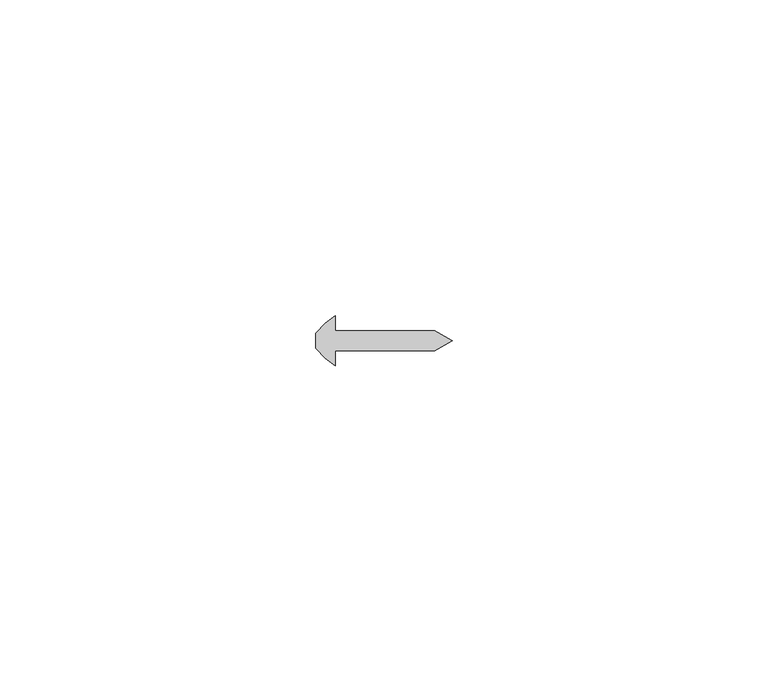
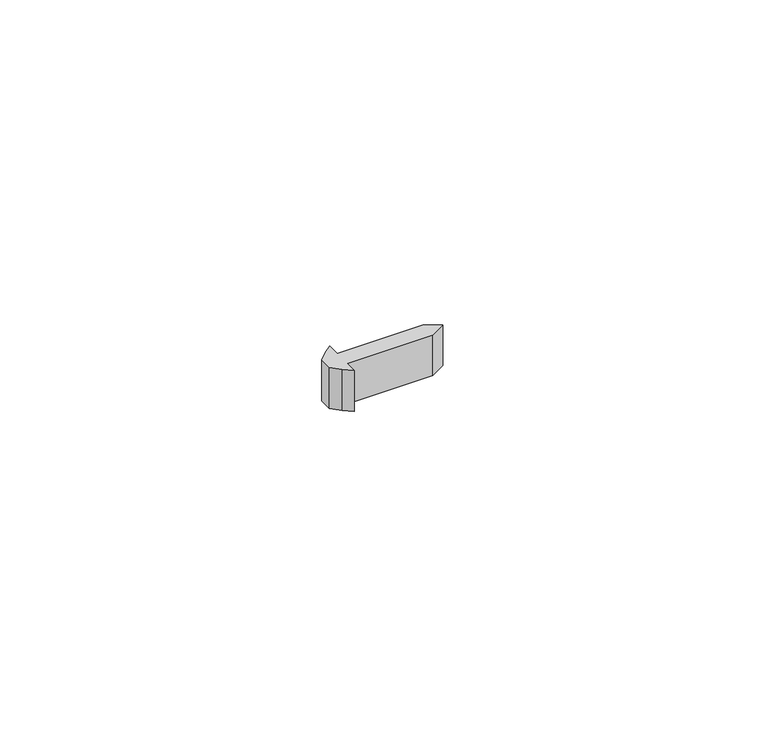
"""IFC4 building model written with IfcOpenShell, lengths in millimetres: proxy geometry, Generic Models 7:Generic Models 1:3:Generic Models 1:3 : Generic Models 7:Generic Models 1:305549:3:Generic Models 1:3:Generic Models 1:3 : Generic Models 7:Generic Models 1:305549:3 : Generic Models 7:Generic Models 1:3:Generic Models 1:3 : Generic Models 7:Generic Models 1:305549:301244:67 : Generic Models 7:Generic Models 1:3:Generic Models 1:3 : Generic Models 7:Generic Models 1:305549:3:Generic Models 1:3:Generic Models 1:3 : Generic Models 7:Generic Models 1:305549:3 : Generic Models 7:Generic Models 1:3:Generic Models 1:3 : Generic Models 7:Generic Models 1:305549:301244:308848."""

from ifc_helpers import new_model, si_unit, frame, origin, place, context, project, spatial, polyline, outline, extrude, source, transform, mapped, element, save


def generic_models_e5c60fd0(model_context):
    return source(origin(), model_context, "Body", "SweptSolid", [
        extrude(outline(polyline([(560281.5242239, -530659.7288841), (560281.5242239, -530662.1101341), (560279.9971659, -530660.8919386), (560278.4452757, -530659.3400484), (560278.4452757, -530656.9427199), (560279.9971659, -530655.3908297), (560281.5242239, -530654.1726341), (560281.5242239, -530656.5538841), (560297.3334794, -530656.5538841), (560300.0831101, -530658.1413841), (560297.3334794, -530659.7288841), (560281.5242239, -530659.7288841)])), frame((0.0, 0.0, 1237.45625), z_axis=(0.0, 0.0, 1.0), x_axis=(1.0, 0.0, 0.0)), (0.0, 0.0, 1.0), 7.9375),
    ])


if __name__ == "__main__":
    model = new_model("IFC4")
    model_context = context("Model", 3, world=origin())
    ifc_project = project(units=[si_unit("LENGTHUNIT", "METRE", prefix="MILLI")], contexts=[model_context])
    site = spatial("IfcSite", under=ifc_project)
    building = spatial("IfcBuilding", under=site)
    placement = place(None, origin())
    generic_models_shape = generic_models_e5c60fd0(model_context)
    element("IfcBuildingElementProxy", 1, Name="Generic Models 7:Generic Models 1:3:Generic Models 1:3 : Generic Models 7:Generic Models 1:305549:3:Generic Models 1:3:Generic Models 1:3 : Generic Models 7:Generic Models 1:305549:3 : Generic Models 7:Generic Models 1:3:Generic Models 1:3 : Generic Models 7:Generic Models 1:305549:301244:67 : Generic Models 7:Generic Models 1:3:Generic Models 1:3 : Generic Models 7:Generic Models 1:305549:3:Generic Models 1:3:Generic Models 1:3 : Generic Models 7:Generic Models 1:305549:3 : Generic Models 7:Generic Models 1:3:Generic Models 1:3 : Generic Models 7:Generic Models 1:305549:301244:308848", ObjectType="Generic Models 7:Generic Models 1:3:Generic Models 1:3 : Generic Models 7:Generic Models 1:305549:3:Generic Models 1:3:Generic Models 1:3 : Generic Models 7:Generic Models 1:305549:3 : Generic Models 7:Generic Models 1:3:Generic Models 1:3 : Generic Models 7:Generic Models 1:305549:301244:67 : Generic Models 7:Generic Models 1:3:Generic Models 1:3 : Generic Models 7:Generic Models 1:305549:3:Generic Models 1:3:Generic Models 1:3 : Generic Models 7:Generic Models 1:305549:3 : Generic Models 7:Generic Models 1:3:Generic Models 1:3 : Generic Models 7:Generic Models 1:305549:301244:308848", at=placement, inside=building, context=model_context, shape_type="MappedRepresentation", body=[
        mapped(generic_models_shape, transform((0.0, 0.0, 0.0), x_axis=(1.0, 0.0, 0.0), y_axis=(0.0, 1.0, 0.0), z_axis=(0.0, 0.0, 1.0))),
    ])
    save(model, "model.ifc")

# Revit data of these elements
# Type "Generic Models 7:Generic Models 1:3:Generic Models 1:3 : Generic Models 7:Generic Models 1:305549:3:Generic Models 1:3:Generic Models 1:3 : Generic Models 7:Generic Models 1:305549:3 : Generic Models 7:Generic Models 1:3:Generic Models 1:3 : Generic Models 7:Generic Models 1:305549:301244:67 : Generic Models 7:Generic Models 1:3:Generic Models 1:3 : Generic Models 7:Generic Models 1:305549:3:Generic Models 1:3:Generic Models 1:3 : Generic Models 7:Generic Models 1:305549:3 : Generic Models 7:Generic Models 1:3:Generic Models 1:3 : Generic Models 7:Generic Models 1:305549:301244:308848"
#   NameOverride = "Generic Models 7:Generic Models 1:3:Generic Models 1:3 : Generic Models 7:Generic Models 1:305549:3:Generic Models 1:3:Generic Models 1:3 : Generic Models 7:Generic Models 1:305549:3 : Generic Models 7:Generic Models 1:3:Generic Models 1:3 : Generic Models 7:Generic Models 1:305549:301244:308848"
#   ObjectTypeOverride = "Generic Models 1:3:Generic Models 1:3 : Generic Models 7:Generic Models 1:305549:3 : Generic Models 7:Generic Models 1:3:Generic Models 1:3 : Generic Models 7:Generic Models 1:305549:301244"
#   Reference = "Generic Models 1"
#   Tag = "308848"
# Element 1 (IfcBuildingElementProxy, "Generic Models 7:Generic Models 1:3:Generic Models 1:3 : Generic Models 7:Generic Models 1:305549:3:Generic Models 1:3:Generic Models 1:3 : Generic Models 7:Generic Models 1:305549:3 : Generic Models 7:Generic Models 1:3:Generic Models 1:3 : Generic Models 7:Generic Models 1:305549:301244:67 : Generic Models 7:Generic Models 1:3:Generic Models 1:3 : Generic Models 7:Generic Models 1:305549:3:Generic Models 1:3:Generic Models 1:3 : Generic Models 7:Generic Models 1:305549:3 : Generic Models 7:Generic Models 1:3:Generic Models 1:3 : Generic Models 7:Generic Models 1:305549:301244:308848")
#   Materials on its faces: "FASTENERS (T.B.D)"
# Materials
#   "FASTENERS (T.B.D)": class "Generic", colour RGB 120 120 120, transparency 0, Cost = 0
